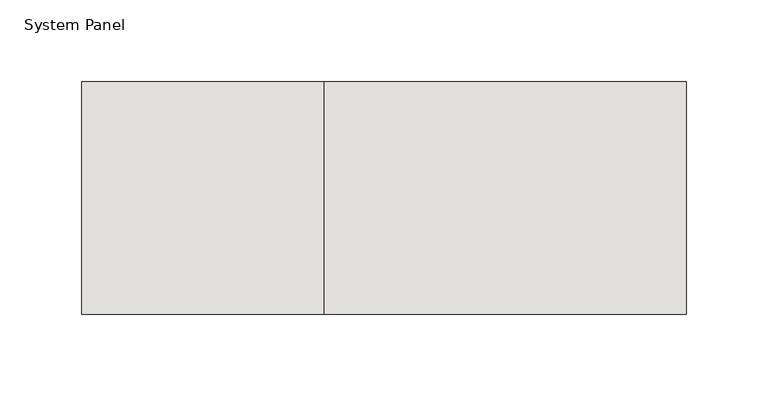
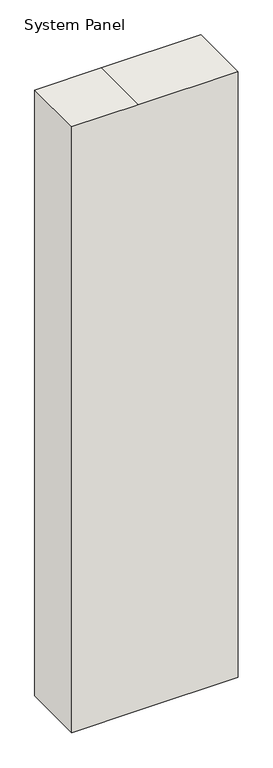
"""IFC4 building model written with IfcOpenShell, lengths in millimetres: wall geometry, System Panel : NLRS_21_CWP_hsb-vulling minerale wol 142 _gen_rsf."""

from ifc_helpers import new_model, si_unit, frame, origin, place, context, project, spatial, polyline, outline, extrude, source, transform, mapped, element, save


def system_panel_d55a1cbf(model_context):
    return source(origin(), model_context, "Body", "SweptSolid", [
        extrude(outline(polyline([(0.0, -184.5), (0.0, -36.3441061), (0.0, 184.5), (1421.0, 184.5), (1421.0, -36.3441061), (1421.0, -184.5), (0.0, -184.5)])), frame((0.0, -71.0, 0.0), z_axis=(0.0, 1.0, 0.0), x_axis=(0.0, 0.0, 1.0)), (0.0, 0.0, 1.0), 142.0),
    ])


if __name__ == "__main__":
    model = new_model("IFC4")
    model_context = context("Model", 3, world=origin())
    ifc_project = project(units=[si_unit("LENGTHUNIT", "METRE", prefix="MILLI")], contexts=[model_context])
    site = spatial("IfcSite", under=ifc_project)
    building = spatial("IfcBuilding", under=site)
    placement = place(None, origin())
    system_panel_shape = system_panel_d55a1cbf(model_context)
    element("IfcWall", 1, ObjectType="System Panel : NLRS_21_CWP_hsb-vulling minerale wol 142 _gen_rsf", at=placement, inside=building, context=model_context, shape_type="MappedRepresentation", body=[
        mapped(system_panel_shape, transform((0.0, 0.0, 0.0), x_axis=(1.0, 0.0, 0.0), y_axis=(0.0, 1.0, 0.0), z_axis=(0.0, 0.0, 1.0))),
    ])
    save(model, "model.ifc")

# Revit data of these elements
# Type "System Panel : NLRS_21_CWP_hsb-vulling minerale wol 142 _gen_rsf"
#   Type IfcGUID = "07M7mRoiH1CR8m_RSKIwpC"
#   Assembly Code = "21.23"
#   IfcExportAs = "IfcWall"
# Element 1 (IfcWall, "System Panel : NLRS_21_CWP_hsb-vulling minerale wol 142 _gen_rsf")
#   Materials on its faces: "NLRS_m1_isolatie minerale wol_gen_rsf"
# Materials
#   "NLRS_m1_isolatie minerale wol_gen_rsf": class "M - Anorganische materialen", colour RGB 200 200 140, transparency 0, Keynote = "m1", Manufacturer = "Revit Standards Foundation", URL = "www.revitstandards.org", Description = "isolatie minerale wol", Cost = 0
